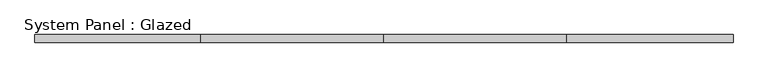
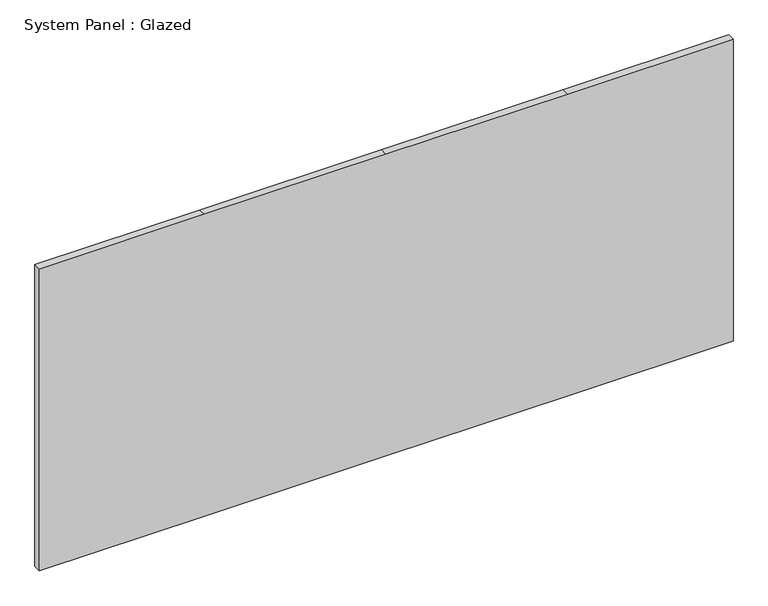
"""IFC4 building model written with IfcOpenShell, lengths in millimetres: plate geometry, System Panel : Glazed."""

from ifc_helpers import new_model, si_unit, frame, origin, place, context, project, spatial, polyline, outline, extrude, source, transform, mapped, element, save


def system_panel_glazed_67c5d381(model_context):
    return source(origin(), model_context, "Body", "SweptSolid", [
        extrude(outline(polyline([(0.0, -2291.0187644), (0.0, -1202.0187644), (0.0, -2.0187644), (0.0, 1197.9812356), (0.0, 2291.0187644), (2110.0, 2291.0187644), (2110.0, 1197.9812356), (2110.0, -2.0187644), (2110.0, -1202.0187644), (2110.0, -2291.0187644), (0.0, -2291.0187644)])), frame((0.0, -25.0, 0.0), z_axis=(0.0, 1.0, 0.0), x_axis=(0.0, 0.0, 1.0)), (0.0, 0.0, 1.0), 50.0),
    ])


if __name__ == "__main__":
    model = new_model("IFC4")
    model_context = context("Model", 3, world=origin())
    ifc_project = project(units=[si_unit("LENGTHUNIT", "METRE", prefix="MILLI")], contexts=[model_context])
    site = spatial("IfcSite", under=ifc_project)
    building = spatial("IfcBuilding", under=site)
    placement = place(None, origin())
    system_panel_glazed_shape = system_panel_glazed_67c5d381(model_context)
    element("IfcPlate", 1, ObjectType="System Panel : Glazed", at=placement, inside=building, context=model_context, shape_type="MappedRepresentation", body=[
        mapped(system_panel_glazed_shape, transform((0.0, 0.0, 0.0), x_axis=(1.0, 0.0, 0.0), y_axis=(0.0, 1.0, 0.0), z_axis=(0.0, 0.0, 1.0))),
    ])
    save(model, "model.ifc")

# Revit data of these elements
# Type "System Panel : Glazed"
#   Type Mark = "CW-GLASS"
# Element 1 (IfcPlate, "System Panel : Glazed")
#   Materials on its faces: "Glass_Clear"
# Materials
#   "Glass_Clear": class "Glass", colour RGB 128 128 255, transparency 0.8, Comments = "Rendering appearance not upgraded ", Cost = 0
